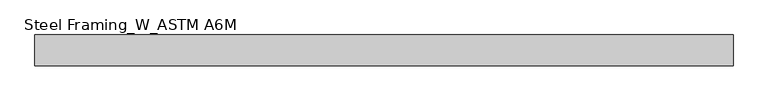
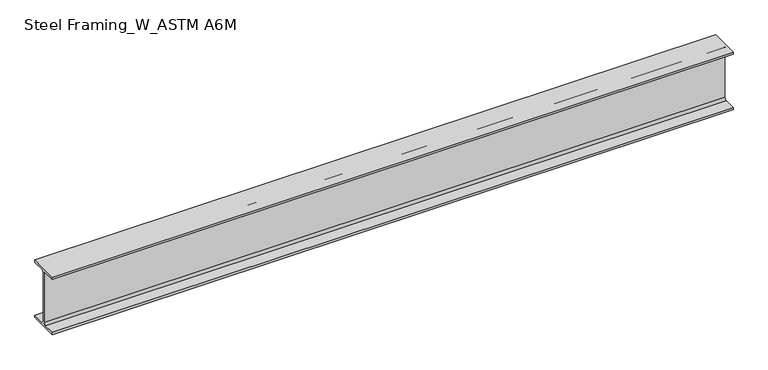
"""IFC4 building model written with IfcOpenShell, lengths in millimetres: beam geometry, Steel Framing_W_ASTM A6M : H_SB_AR_S02_W200x22.5_B7."""

import ifcopenshell
import ifcopenshell.guid

model = None  # the IFC model being written
_history = None  # IfcOwnerHistory: only IFC2X3 demands one
_inside = {}  # id of a spatial element -> (the spatial element, [elements in it])
_under = {}  # id of a project, library or spatial element -> (it, [spatial elements below it])
_declared = {}  # id of a project -> (the project, [libraries it declares])
_typed = {}  # id of a type object -> (the type object, [elements of that type])
_made_of = {}  # id of a material, layer set ... -> (it, [elements and type objects made of it])


def new_model(schema):
    """Start an empty IFC model of exactly this schema.

    Asked for "IFC4X3", IfcOpenShell would pick the latest addendum, in which some entities
    have other attributes; the version numbers below select the first issue.
    IFC2X3 requires an IfcOwnerHistory on every rooted entity: one is made here for all.
    """
    global model, _history
    if schema == "IFC4X3":
        model = ifcopenshell.file(schema_version=(4, 3, 0, 0))
    else:
        model = ifcopenshell.file(schema=schema)
    _inside.clear()
    _under.clear()
    _declared.clear()
    _typed.clear()
    _made_of.clear()
    _history = None
    if model.schema == "IFC2X3":
        org = make("IfcOrganization", Name="unknown")
        user = make(
            "IfcPersonAndOrganization",
            ThePerson=make("IfcPerson", FamilyName="unknown"),
            TheOrganization=org,
        )
        app = make(
            "IfcApplication",
            ApplicationDeveloper=org,
            Version="unknown",
            ApplicationFullName="unknown",
            ApplicationIdentifier="unknown",
        )
        _history = make(
            "IfcOwnerHistory",
            OwningUser=user,
            OwningApplication=app,
            ChangeAction="ADDED",
            CreationDate=0,
        )
    return model


def make(cls, **values):
    """One entity of the class cls with the attributes given. An attribute that is None is left unset."""
    return model.create_entity(
        cls, **{name: value for name, value in values.items() if value is not None}
    )


def rooted(cls, **values):
    """An entity with a GlobalId (a new one), such as an element, a storey or a relation."""
    return make(cls, GlobalId=ifcopenshell.guid.new(), OwnerHistory=_history, **values)


def si_unit(unit_type, name, prefix=None):
    """IfcSIUnit, for example si_unit("LENGTHUNIT", "METRE", prefix="MILLI")."""
    return make("IfcSIUnit", UnitType=unit_type, Prefix=prefix, Name=name)


def assignment(units):
    """IfcUnitAssignment: the units of a project."""
    return None if units is None else make("IfcUnitAssignment", Units=units)


def point(xyz):
    """IfcCartesianPoint."""
    return None if xyz is None else make("IfcCartesianPoint", Coordinates=xyz)


def direction(xyz):
    """IfcDirection."""
    return None if xyz is None else make("IfcDirection", DirectionRatios=xyz)


def frame(location, z_axis=None, x_axis=None):
    """IfcAxis2Placement3D, a coordinate frame: its origin and axes. An axis left out is left unset."""
    return make(
        "IfcAxis2Placement3D",
        Location=point(location),
        Axis=direction(z_axis),
        RefDirection=direction(x_axis),
    )


def frame_2d(location, x_axis=None):
    """IfcAxis2Placement2D, a coordinate frame in the plane: its origin and x axis."""
    return make(
        "IfcAxis2Placement2D", Location=point(location), RefDirection=direction(x_axis)
    )


def origin():
    """The frame at (0, 0, 0) with its axes left unset."""
    return frame((0.0, 0.0, 0.0))


def place(relative_to, where):
    """IfcLocalPlacement: puts the frame where relative to a parent placement (None: the world)."""
    return make(
        "IfcLocalPlacement", PlacementRelTo=relative_to, RelativePlacement=where
    )


def context(
    kind, dimensions, precision=None, world=None, true_north=None, identifier=None
):
    """IfcGeometricRepresentationContext, for example the 3D "Model" context."""
    return make(
        "IfcGeometricRepresentationContext",
        ContextIdentifier=identifier,
        ContextType=kind,
        CoordinateSpaceDimension=dimensions,
        Precision=precision,
        WorldCoordinateSystem=world,
        TrueNorth=true_north,
    )


def project(units=None, contexts=None):
    """IfcProject with its units and contexts."""
    return rooted(
        "IfcProject",
        Name="project",
        RepresentationContexts=contexts,
        UnitsInContext=assignment(units),
    )


def spatial(cls, under=None, at=None, **own):
    """A site, building, storey or space (cls), placed at a placement, below another one or the project."""
    s = rooted(cls, ObjectPlacement=at, **own)
    if under is not None:
        _under.setdefault(under.id(), (under, []))[1].append(s)
    return s


def polyline(points):
    """IfcPolyline through the points."""
    return make("IfcPolyline", Points=[point(p) for p in points])


def circle_curve(where, radius):
    """IfcCircle in the frame where."""
    return make("IfcCircle", Position=where, Radius=radius)


def trimmed(basis, trim1, trim2, sense, master):
    """IfcTrimmedCurve: the piece of a basis curve between two trims."""
    return make(
        "IfcTrimmedCurve",
        BasisCurve=basis,
        Trim1=trim1,
        Trim2=trim2,
        SenseAgreement=sense,
        MasterRepresentation=master,
    )


def segment(curve, same_sense, transition):
    """IfcCompositeCurveSegment."""
    return make(
        "IfcCompositeCurveSegment",
        Transition=transition,
        SameSense=same_sense,
        ParentCurve=curve,
    )


def composite_curve(segments, self_intersect=None):
    """IfcCompositeCurve: segments joined end to end."""
    return make("IfcCompositeCurve", Segments=segments, SelfIntersect=self_intersect)


def outline(outer, holes=None, kind="AREA"):
    """IfcArbitraryClosedProfileDef: a profile drawn as a closed curve; with holes, ...WithVoids."""
    if holes is None:
        return make("IfcArbitraryClosedProfileDef", ProfileType=kind, OuterCurve=outer)
    return make(
        "IfcArbitraryProfileDefWithVoids",
        ProfileType=kind,
        OuterCurve=outer,
        InnerCurves=holes,
    )


def extrude(swept, where, along, depth):
    """IfcExtrudedAreaSolid: the profile swept, set in the frame where, extruded along a direction by depth."""
    return make(
        "IfcExtrudedAreaSolid",
        SweptArea=swept,
        Position=where,
        ExtrudedDirection=direction(along),
        Depth=depth,
    )


def shape(context_of_items, identifier, shape_type, items):
    """IfcShapeRepresentation: the items that make up one representation, for example the "Body"."""
    return make(
        "IfcShapeRepresentation",
        ContextOfItems=context_of_items,
        RepresentationIdentifier=identifier,
        RepresentationType=shape_type,
        Items=items,
    )


def source(mapping_origin, context_of_items, identifier, shape_type, items):
    """IfcRepresentationMap: a shape defined once, which mapped items show again and again."""
    return make(
        "IfcRepresentationMap",
        MappingOrigin=mapping_origin,
        MappedRepresentation=shape(context_of_items, identifier, shape_type, items),
    )


def transform(
    local_origin,
    x_axis=None,
    y_axis=None,
    z_axis=None,
    scale=None,
    scale2=None,
    scale3=None,
    uniform=True,
):
    """IfcCartesianTransformationOperator3D, or its non-uniform kind. x_axis, y_axis, z_axis: its Axis1, 2, 3."""
    if uniform:
        return make(
            "IfcCartesianTransformationOperator3D",
            Axis1=direction(x_axis),
            Axis2=direction(y_axis),
            LocalOrigin=point(local_origin),
            Scale=scale,
            Axis3=direction(z_axis),
        )
    return make(
        "IfcCartesianTransformationOperator3DnonUniform",
        Axis1=direction(x_axis),
        Axis2=direction(y_axis),
        LocalOrigin=point(local_origin),
        Scale=scale,
        Axis3=direction(z_axis),
        Scale2=scale2,
        Scale3=scale3,
    )


def mapped(mapping_source, mapping_target):
    """IfcMappedItem: shows the shape of a source again, moved by a transform."""
    return make(
        "IfcMappedItem", MappingSource=mapping_source, MappingTarget=mapping_target
    )


def made_of(thing, what):
    """Note that an element or type object is made of a material, layer set ...; save() writes the relation."""
    if what is not None:
        _made_of.setdefault(what.id(), (what, []))[1].append(thing)
    return thing


def element(
    cls,
    number,
    at=None,
    inside=None,
    cuts=None,
    type_object=None,
    material=None,
    context=None,
    identifier="Body",
    shape_type=None,
    held_by="IfcProductDefinitionShape",
    body=None,
    shapes=None,
    **own,
):
    """One element of the class cls, such as IfcWall. Its Tag is "e" and its number.

    at: its placement. inside: the storey or other place that contains it. cuts: it is an
    opening in that element (IfcRelVoidsElement). A single representation is given by context,
    identifier, shape_type and body (its items); several are given by shapes. held_by: the class
    of the entity that holds the representations. save() writes the other relations.
    """
    e = rooted(cls, Tag="e%d" % number, ObjectPlacement=at, **own)
    if body is not None:
        shapes = [shape(context, identifier, shape_type, body)]
    if shapes is not None:
        e.Representation = make(held_by, Representations=shapes)
    if inside is not None:
        _inside.setdefault(inside.id(), (inside, []))[1].append(e)
    if cuts is not None:
        rooted(
            "IfcRelVoidsElement", RelatingBuildingElement=cuts, RelatedOpeningElement=e
        )
    if type_object is not None:
        _typed.setdefault(type_object.id(), (type_object, []))[1].append(e)
    return made_of(e, material)


def aggregate(whole, parts):
    """IfcRelAggregates: a whole, such as a stair, and the parts it consists of."""
    return rooted("IfcRelAggregates", RelatingObject=whole, RelatedObjects=parts)


def save(model, path):
    """Write the relations noted so far, then the file.

    IfcRelAggregates (storeys below a building ...), IfcRelContainedInSpatialStructure (elements
    in a storey), IfcRelDefinesByType, IfcRelAssociatesMaterial and IfcRelDeclares: one each for
    every whole, place, type object, material and project.
    """
    for whole, parts in _under.values():
        aggregate(whole, parts)
    for where, things in _inside.values():
        rooted(
            "IfcRelContainedInSpatialStructure",
            RelatedElements=things,
            RelatingStructure=where,
        )
    for kind, things in _typed.values():
        rooted("IfcRelDefinesByType", RelatedObjects=things, RelatingType=kind)
    for what, things in _made_of.values():
        rooted("IfcRelAssociatesMaterial", RelatedObjects=things, RelatingMaterial=what)
    for by, libraries in _declared.values():
        rooted("IfcRelDeclares", RelatingContext=by, RelatedDefinitions=libraries)
    model.write(path)


def steel_framing_w_astm_a6m_683fa1ff(model_context):
    return source(origin(), model_context, "Body", "SweptSolid", [
        extrude(outline(composite_curve([segment(polyline([(51.0, -95.0), (51.0, -103.0), (-51.0, -103.0), (-51.0, -95.0), (-10.71, -95.0)]), True, "CONTINUOUS"), segment(trimmed(circle_curve(frame_2d((-10.71, -87.4)), 7.6), [point((-10.71, -95.0))], [point((-3.11, -87.4))], True, "CARTESIAN"), True, "CONTINUOUS"), segment(polyline([(-3.11, -87.4), (-3.11, 87.4)]), True, "CONTINUOUS"), segment(trimmed(circle_curve(frame_2d((-10.71, 87.4)), 7.6), [point((-3.11, 87.4))], [point((-10.71, 95.0))], True, "CARTESIAN"), True, "CONTINUOUS"), segment(polyline([(-10.71, 95.0), (-51.0, 95.0), (-51.0, 103.0), (51.0, 103.0), (51.0, 95.0), (10.71, 95.0)]), True, "CONTINUOUS"), segment(trimmed(circle_curve(frame_2d((10.71, 87.4)), 7.6), [point((10.71, 95.0))], [point((3.11, 87.4))], True, "CARTESIAN"), True, "CONTINUOUS"), segment(polyline([(3.11, 87.4), (3.11, -87.4)]), True, "CONTINUOUS"), segment(trimmed(circle_curve(frame_2d((10.71, -87.4)), 7.6), [point((3.11, -87.4))], [point((10.71, -95.0))], True, "CARTESIAN"), True, "CONTINUOUS"), segment(polyline([(10.71, -95.0), (51.0, -95.0)]), True, "CONTINUOUS")], self_intersect=False)), frame((-1151.8, 0.0, 0.0), z_axis=(1.0, 0.0, 0.0), x_axis=(0.0, 1.0, 0.0)), (0.0, 0.0, 1.0), 2303.6),
    ])


if __name__ == "__main__":
    model = new_model("IFC4")
    model_context = context("Model", 3, world=origin())
    ifc_project = project(units=[si_unit("LENGTHUNIT", "METRE", prefix="MILLI")], contexts=[model_context])
    site = spatial("IfcSite", under=ifc_project)
    building = spatial("IfcBuilding", under=site)
    placement = place(None, origin())
    steel_framing_w_astm_a6m_shape = steel_framing_w_astm_a6m_683fa1ff(model_context)
    element("IfcBeam", 1, ObjectType="Steel Framing_W_ASTM A6M : H_SB_AR_S02_W200x22.5_B7", at=placement, inside=building, context=model_context, shape_type="MappedRepresentation", body=[
        mapped(steel_framing_w_astm_a6m_shape, transform((0.0, 0.0, 0.0), x_axis=(1.0, 0.0, 0.0), y_axis=(0.0, 1.0, 0.0), z_axis=(0.0, 0.0, 1.0))),
    ])
    save(model, "model.ifc")

# Revit data of these elements
# Type "Steel Framing_W_ASTM A6M : H_SB_AR_S02_W200x22.5_B7"
#   Section Name Key = "W8x15"
#   Width = 10.2 cm
#   Web Thickness = 0.622 cm
#   Web Fillet = 0.76 cm
#   Warping Constant = 13900.0 cm⁶
#   Torsional Moment of Inertia = 5.70 cm⁴
#   Section Area = 28.6 cm²
#   Plastic Modulus weak axis = 43.8 cm³
#   Plastic Modulus strong axis = 223.0 cm³
#   Perimeter = 0.795 m²/m
#   Nominal Weight = 22.50 kgf/m
#   Moment of Inertia weak axis = 142.00 cm⁴
#   Moment of Inertia strong axis = 2000.00 cm⁴
#   Height = 20.6 cm
#   Flange Thickness = 0.8 cm
#   Elastic Modulus weak axis = 27.9 cm³
#   Elastic Modulus strong axis = 193.0 cm³
#   Centroid Vertical = 10.3 cm
#   Centroid Horizontal = 5.1 cm
#   Length [instance default] = 1500 mm
#   Structural Material [instance default] = Steel, 45-345
#   Bolt Spacing = 0
#   Assembly Code = ""
# Element 1 (IfcBeam, "Steel Framing_W_ASTM A6M : H_SB_AR_S02_W200x22.5_B7")
#   Materials on its faces: "Steel, 45-345"
# Materials
#   "Steel, 45-345": class "Metal", colour RGB 189 187 185, transparency 0, Description = "Steel 345 MPa", Cost = 0
